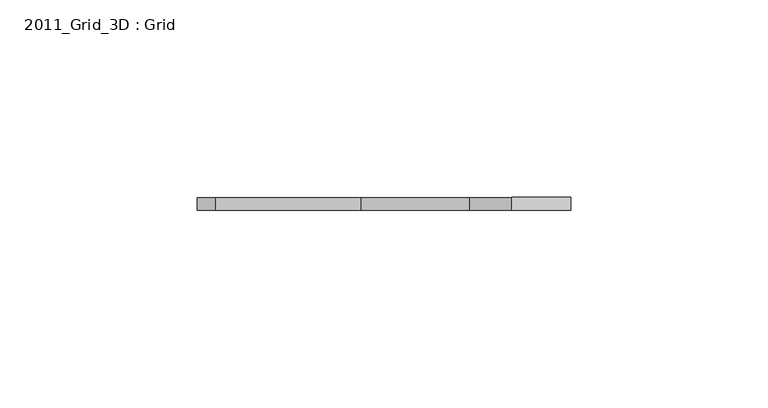
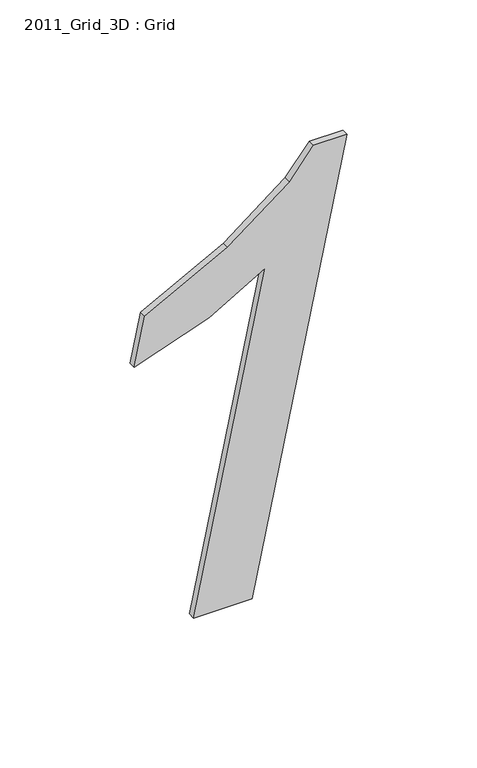
"""IFC4 building model written with IfcOpenShell, lengths in millimetres: proxy geometry, 2011_Grid_3D : Grid."""

from ifc_helpers import new_model, si_unit, frame, origin, place, context, project, spatial, polyline, outline, extrude, source, transform, mapped, element, save


def proxy_2011_grid_3d_grid_89aafc61(model_context):
    return source(origin(), model_context, "Body", "SweptSolid", [
        extrude(outline(polyline([(-101.6, 29940.1966257), (-101.6, 29966.0233601), (101.4447294, 30008.2086786), (101.4447294, 29993.38681), (88.0108618, 29982.6298016), (67.0173455, 29955.1919945), (47.5109731, 29918.4347517), (25.3029559, 29913.7750337), (36.729179, 29947.0498811), (51.3775476, 29971.9223647), (-101.6, 29940.1966257)])), frame((0.0, -3.175, 0.0), z_axis=(0.0, 1.0, 0.0), x_axis=(0.0, 0.0, 1.0)), (0.0, 0.0, 1.0), 3.175),
    ])


if __name__ == "__main__":
    model = new_model("IFC4")
    model_context = context("Model", 3, world=origin())
    ifc_project = project(units=[si_unit("LENGTHUNIT", "METRE", prefix="MILLI")], contexts=[model_context])
    site = spatial("IfcSite", under=ifc_project)
    building = spatial("IfcBuilding", under=site)
    placement = place(None, origin())
    proxy_2011_grid_3d_grid_shape = proxy_2011_grid_3d_grid_89aafc61(model_context)
    element("IfcBuildingElementProxy", 1, Name="2011_Grid_3D : Grid", ObjectType="2011_Grid_3D : Grid", at=placement, inside=building, context=model_context, shape_type="MappedRepresentation", body=[
        mapped(proxy_2011_grid_3d_grid_shape, transform((0.0, 0.0, 0.0), x_axis=(1.0, 0.0, 0.0), y_axis=(0.0, 1.0, 0.0), z_axis=(0.0, 0.0, 1.0))),
    ])
    save(model, "model.ifc")

# Revit data of these elements
# Type "2011_Grid_3D : Grid"
#   Workplane [instance default] = "LEVEL"
#   Grid [instance default] = "S"
#   t [instance default] = 12' - 6"
#   built-in parameter 1001306 [instance default] = 50 (stored number, unit not read)
#   d [instance default] = 2
#   Symbol At End 2 [instance default] = yes
#   Symbol At End 1 [instance default] = yes
#   Robust [instance default] = yes
#   No of grid markers [instance default] = 3
#   Grid Height Visible = yes
#   Height = 0
#   Assembly Code = ""
# Element 1 (IfcBuildingElementProxy, "2011_Grid_3D : Grid")
#   Workplane = "1"
#   Grid = "5"
#   t = 12' - 2 1/4"
#   built-in parameter 1001306 = 97.5 (stored number, unit not read)
#   d = 4
#   Robust = no
#   No of grid markers = 5
#   Materials on its faces: "Letter"
# Materials
#   "Letter": class "Unassigned", colour RGB 178 187 30, transparency 0, Comments = "Rendering appearance not upgraded "
